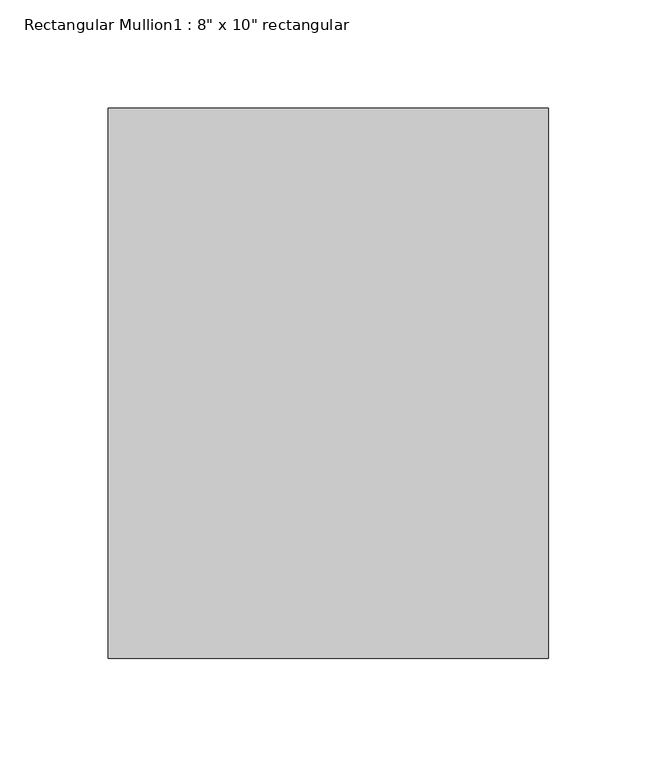
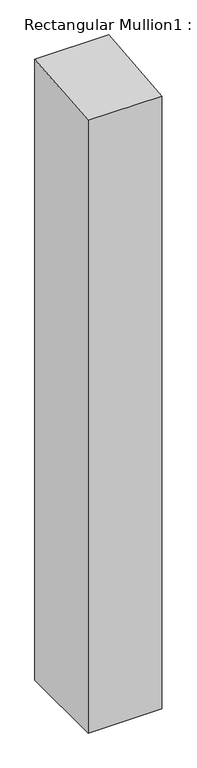
"""IFC4 building model written with IfcOpenShell, lengths in millimetres: member geometry."""

import ifcopenshell
import ifcopenshell.guid

model = None  # the IFC model being written
_history = None  # IfcOwnerHistory: only IFC2X3 demands one
_inside = {}  # id of a spatial element -> (the spatial element, [elements in it])
_under = {}  # id of a project, library or spatial element -> (it, [spatial elements below it])
_declared = {}  # id of a project -> (the project, [libraries it declares])
_typed = {}  # id of a type object -> (the type object, [elements of that type])
_made_of = {}  # id of a material, layer set ... -> (it, [elements and type objects made of it])


def new_model(schema):
    """Start an empty IFC model of exactly this schema.

    Asked for "IFC4X3", IfcOpenShell would pick the latest addendum, in which some entities
    have other attributes; the version numbers below select the first issue.
    IFC2X3 requires an IfcOwnerHistory on every rooted entity: one is made here for all.
    """
    global model, _history
    if schema == "IFC4X3":
        model = ifcopenshell.file(schema_version=(4, 3, 0, 0))
    else:
        model = ifcopenshell.file(schema=schema)
    _inside.clear()
    _under.clear()
    _declared.clear()
    _typed.clear()
    _made_of.clear()
    _history = None
    if model.schema == "IFC2X3":
        org = make("IfcOrganization", Name="unknown")
        user = make(
            "IfcPersonAndOrganization",
            ThePerson=make("IfcPerson", FamilyName="unknown"),
            TheOrganization=org,
        )
        app = make(
            "IfcApplication",
            ApplicationDeveloper=org,
            Version="unknown",
            ApplicationFullName="unknown",
            ApplicationIdentifier="unknown",
        )
        _history = make(
            "IfcOwnerHistory",
            OwningUser=user,
            OwningApplication=app,
            ChangeAction="ADDED",
            CreationDate=0,
        )
    return model


def make(cls, **values):
    """One entity of the class cls with the attributes given. An attribute that is None is left unset."""
    return model.create_entity(
        cls, **{name: value for name, value in values.items() if value is not None}
    )


def rooted(cls, **values):
    """An entity with a GlobalId (a new one), such as an element, a storey or a relation."""
    return make(cls, GlobalId=ifcopenshell.guid.new(), OwnerHistory=_history, **values)


def si_unit(unit_type, name, prefix=None):
    """IfcSIUnit, for example si_unit("LENGTHUNIT", "METRE", prefix="MILLI")."""
    return make("IfcSIUnit", UnitType=unit_type, Prefix=prefix, Name=name)


def assignment(units):
    """IfcUnitAssignment: the units of a project."""
    return None if units is None else make("IfcUnitAssignment", Units=units)


def point(xyz):
    """IfcCartesianPoint."""
    return None if xyz is None else make("IfcCartesianPoint", Coordinates=xyz)


def direction(xyz):
    """IfcDirection."""
    return None if xyz is None else make("IfcDirection", DirectionRatios=xyz)


def frame(location, z_axis=None, x_axis=None):
    """IfcAxis2Placement3D, a coordinate frame: its origin and axes. An axis left out is left unset."""
    return make(
        "IfcAxis2Placement3D",
        Location=point(location),
        Axis=direction(z_axis),
        RefDirection=direction(x_axis),
    )


def origin():
    """The frame at (0, 0, 0) with its axes left unset."""
    return frame((0.0, 0.0, 0.0))


def place(relative_to, where):
    """IfcLocalPlacement: puts the frame where relative to a parent placement (None: the world)."""
    return make(
        "IfcLocalPlacement", PlacementRelTo=relative_to, RelativePlacement=where
    )


def context(
    kind, dimensions, precision=None, world=None, true_north=None, identifier=None
):
    """IfcGeometricRepresentationContext, for example the 3D "Model" context."""
    return make(
        "IfcGeometricRepresentationContext",
        ContextIdentifier=identifier,
        ContextType=kind,
        CoordinateSpaceDimension=dimensions,
        Precision=precision,
        WorldCoordinateSystem=world,
        TrueNorth=true_north,
    )


def project(units=None, contexts=None):
    """IfcProject with its units and contexts."""
    return rooted(
        "IfcProject",
        Name="project",
        RepresentationContexts=contexts,
        UnitsInContext=assignment(units),
    )


def spatial(cls, under=None, at=None, **own):
    """A site, building, storey or space (cls), placed at a placement, below another one or the project."""
    s = rooted(cls, ObjectPlacement=at, **own)
    if under is not None:
        _under.setdefault(under.id(), (under, []))[1].append(s)
    return s


def polyline(points):
    """IfcPolyline through the points."""
    return make("IfcPolyline", Points=[point(p) for p in points])


def outline(outer, holes=None, kind="AREA"):
    """IfcArbitraryClosedProfileDef: a profile drawn as a closed curve; with holes, ...WithVoids."""
    if holes is None:
        return make("IfcArbitraryClosedProfileDef", ProfileType=kind, OuterCurve=outer)
    return make(
        "IfcArbitraryProfileDefWithVoids",
        ProfileType=kind,
        OuterCurve=outer,
        InnerCurves=holes,
    )


def extrude(swept, where, along, depth):
    """IfcExtrudedAreaSolid: the profile swept, set in the frame where, extruded along a direction by depth."""
    return make(
        "IfcExtrudedAreaSolid",
        SweptArea=swept,
        Position=where,
        ExtrudedDirection=direction(along),
        Depth=depth,
    )


def shape(context_of_items, identifier, shape_type, items):
    """IfcShapeRepresentation: the items that make up one representation, for example the "Body"."""
    return make(
        "IfcShapeRepresentation",
        ContextOfItems=context_of_items,
        RepresentationIdentifier=identifier,
        RepresentationType=shape_type,
        Items=items,
    )


def source(mapping_origin, context_of_items, identifier, shape_type, items):
    """IfcRepresentationMap: a shape defined once, which mapped items show again and again."""
    return make(
        "IfcRepresentationMap",
        MappingOrigin=mapping_origin,
        MappedRepresentation=shape(context_of_items, identifier, shape_type, items),
    )


def transform(
    local_origin,
    x_axis=None,
    y_axis=None,
    z_axis=None,
    scale=None,
    scale2=None,
    scale3=None,
    uniform=True,
):
    """IfcCartesianTransformationOperator3D, or its non-uniform kind. x_axis, y_axis, z_axis: its Axis1, 2, 3."""
    if uniform:
        return make(
            "IfcCartesianTransformationOperator3D",
            Axis1=direction(x_axis),
            Axis2=direction(y_axis),
            LocalOrigin=point(local_origin),
            Scale=scale,
            Axis3=direction(z_axis),
        )
    return make(
        "IfcCartesianTransformationOperator3DnonUniform",
        Axis1=direction(x_axis),
        Axis2=direction(y_axis),
        LocalOrigin=point(local_origin),
        Scale=scale,
        Axis3=direction(z_axis),
        Scale2=scale2,
        Scale3=scale3,
    )


def mapped(mapping_source, mapping_target):
    """IfcMappedItem: shows the shape of a source again, moved by a transform."""
    return make(
        "IfcMappedItem", MappingSource=mapping_source, MappingTarget=mapping_target
    )


def made_of(thing, what):
    """Note that an element or type object is made of a material, layer set ...; save() writes the relation."""
    if what is not None:
        _made_of.setdefault(what.id(), (what, []))[1].append(thing)
    return thing


def element(
    cls,
    number,
    at=None,
    inside=None,
    cuts=None,
    type_object=None,
    material=None,
    context=None,
    identifier="Body",
    shape_type=None,
    held_by="IfcProductDefinitionShape",
    body=None,
    shapes=None,
    **own,
):
    """One element of the class cls, such as IfcWall. Its Tag is "e" and its number.

    at: its placement. inside: the storey or other place that contains it. cuts: it is an
    opening in that element (IfcRelVoidsElement). A single representation is given by context,
    identifier, shape_type and body (its items); several are given by shapes. held_by: the class
    of the entity that holds the representations. save() writes the other relations.
    """
    e = rooted(cls, Tag="e%d" % number, ObjectPlacement=at, **own)
    if body is not None:
        shapes = [shape(context, identifier, shape_type, body)]
    if shapes is not None:
        e.Representation = make(held_by, Representations=shapes)
    if inside is not None:
        _inside.setdefault(inside.id(), (inside, []))[1].append(e)
    if cuts is not None:
        rooted(
            "IfcRelVoidsElement", RelatingBuildingElement=cuts, RelatedOpeningElement=e
        )
    if type_object is not None:
        _typed.setdefault(type_object.id(), (type_object, []))[1].append(e)
    return made_of(e, material)


def aggregate(whole, parts):
    """IfcRelAggregates: a whole, such as a stair, and the parts it consists of."""
    return rooted("IfcRelAggregates", RelatingObject=whole, RelatedObjects=parts)


def save(model, path):
    """Write the relations noted so far, then the file.

    IfcRelAggregates (storeys below a building ...), IfcRelContainedInSpatialStructure (elements
    in a storey), IfcRelDefinesByType, IfcRelAssociatesMaterial and IfcRelDeclares: one each for
    every whole, place, type object, material and project.
    """
    for whole, parts in _under.values():
        aggregate(whole, parts)
    for where, things in _inside.values():
        rooted(
            "IfcRelContainedInSpatialStructure",
            RelatedElements=things,
            RelatingStructure=where,
        )
    for kind, things in _typed.values():
        rooted("IfcRelDefinesByType", RelatedObjects=things, RelatingType=kind)
    for what, things in _made_of.values():
        rooted("IfcRelAssociatesMaterial", RelatedObjects=things, RelatingMaterial=what)
    for by, libraries in _declared.values():
        rooted("IfcRelDeclares", RelatingContext=by, RelatedDefinitions=libraries)
    model.write(path)


def member_84ccbaea(model_context):
    return source(origin(), model_context, "Body", "SweptSolid", [
        extrude(outline(polyline([(-127.0, -11.9934772), (127.0, 11.9934772), (127.0, -1797.05), (-127.0, -1797.05), (-127.0, -11.9934772)])), frame((-101.6, 0.0, 0.0), z_axis=(1.0, 0.0, 0.0), x_axis=(0.0, 1.0, 0.0)), (0.0, 0.0, 1.0), 203.2),
    ])


if __name__ == "__main__":
    model = new_model("IFC4")
    model_context = context("Model", 3, world=origin())
    ifc_project = project(units=[si_unit("LENGTHUNIT", "METRE", prefix="MILLI")], contexts=[model_context])
    site = spatial("IfcSite", under=ifc_project)
    building = spatial("IfcBuilding", under=site)
    placement = place(None, origin())
    member_shape = member_84ccbaea(model_context)
    element("IfcMember", 1, ObjectType="Rectangular Mullion1 : 8\" x 10\" rectangular", at=placement, inside=building, context=model_context, shape_type="MappedRepresentation", body=[
        mapped(member_shape, transform((0.0, 0.0, 0.0), x_axis=(1.0, 0.0, 0.0), y_axis=(0.0, 1.0, 0.0), z_axis=(0.0, 0.0, 1.0))),
    ])
    save(model, "model.ifc")

# Revit data of these elements
# Type "Rectangular Mullion1 : 8\" x 10\" rectangular"
#   built-in parameter 1007304 = 0.833333 (stored number, unit not read)
#   built-in parameter 1007301 = 0.333333 (stored number, unit not read)
#   built-in parameter 1007300 = 0.333333 (stored number, unit not read)
# Element 1 (IfcMember, "Rectangular Mullion1 : 8\" x 10\" rectangular")
#   Materials on its faces: "support-frame"
# Materials
#   "support-frame": class "Unassigned", colour RGB 233 233 233, transparency 0, Cost = 0
